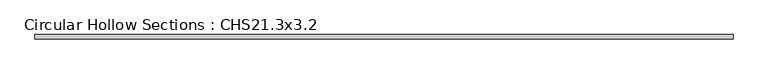
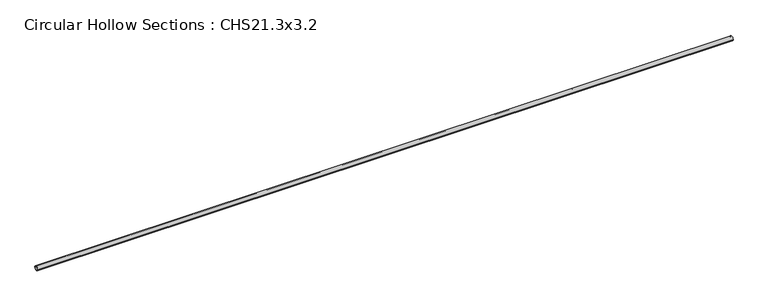
"""IFC4 building model written with IfcOpenShell, lengths in millimetres: member geometry, Circular Hollow Sections : CHS21.3x3.2."""

from ifc_helpers import new_model, si_unit, point, frame, origin, origin_2d, place, context, project, spatial, circle_curve, trimmed, segment, composite_curve, outline, extrude, source, transform, mapped, element, save


def circular_hollow_sections_chs21_3x3_2_132da75c(model_context):
    return source(origin(), model_context, "Body", "SweptSolid", [
        extrude(outline(composite_curve([segment(trimmed(circle_curve(origin_2d(), 10.65), [point((-10.65, 0.0))], [point((10.65, 0.0))], False, "CARTESIAN"), True, "CONTINUOUS"), segment(trimmed(circle_curve(origin_2d(), 10.65), [point((10.65, 0.0))], [point((-10.65, 0.0))], False, "CARTESIAN"), True, "CONTINUOUS")], self_intersect=False), holes=[composite_curve([segment(trimmed(circle_curve(origin_2d(), 7.45), [point((7.45, 0.0))], [point((-7.45, 0.0))], True, "CARTESIAN"), True, "CONTINUOUS"), segment(trimmed(circle_curve(origin_2d(), 7.45), [point((-7.45, 0.0))], [point((7.45, 0.0))], True, "CARTESIAN"), True, "CONTINUOUS")], self_intersect=False)]), frame((-1569.15, 0.0, 0.0), z_axis=(1.0, 0.0, 0.0), x_axis=(0.0, 1.0, 0.0)), (0.0, 0.0, 1.0), 3258.2),
    ])


if __name__ == "__main__":
    model = new_model("IFC4")
    model_context = context("Model", 3, world=origin())
    ifc_project = project(units=[si_unit("LENGTHUNIT", "METRE", prefix="MILLI")], contexts=[model_context])
    site = spatial("IfcSite", under=ifc_project)
    building = spatial("IfcBuilding", under=site)
    placement = place(None, origin())
    circular_hollow_sections_chs21_3x3_2_shape = circular_hollow_sections_chs21_3x3_2_132da75c(model_context)
    element("IfcMember", 1, ObjectType="Circular Hollow Sections : CHS21.3x3.2", at=placement, inside=building, context=model_context, shape_type="MappedRepresentation", body=[
        mapped(circular_hollow_sections_chs21_3x3_2_shape, transform((0.0, 0.0, 0.0), x_axis=(1.0, 0.0, 0.0), y_axis=(0.0, 1.0, 0.0), z_axis=(0.0, 0.0, 1.0))),
    ])
    save(model, "model.ifc")

# Revit data of these elements
# Type "Circular Hollow Sections : CHS21.3x3.2"
#   Section Name Key = "Ch21.3x3.2"
#   Wall Nominal Thickness = 0.32 cm
#   Wall Design Thickness = 0.32 cm
#   Torsional Moment of Inertia = 1.54 cm⁴
#   Torsional Modulus = 1.44 cm³
#   Section Area = 1.82 cm²
#   Plastic Modulus strong axis = 1.06 cm³
#   Perimeter = 0.067 m²/m
#   Nominal Weight = 1.42999 kgf/m
#   Moment of Inertia strong axis = 0.768 cm⁴
#   Length [instance default] = 1500 mm
#   Elastic Modulus strong axis = 0.722 cm³
#   Diameter = 2.13 cm
#   Centroid Vertical = 1.065 cm
#   Centroid Horizontal = 1.065 cm
#   Structural Material [instance default] = Metal - Steel 50-355
#   Type Comments = ""
#   Assembly Code = ""
# Element 1 (IfcMember, "Circular Hollow Sections : CHS21.3x3.2")
#   Structural Material = Metal - Steel 43-275
#   Materials on its faces: "Metal - Steel 43-275"
# Materials
#   "Metal - Steel 50-355": class "Metal", colour RGB 247 247 247, transparency 0, Cost = 0
#   "Metal - Steel 43-275": class "Metal", colour RGB 247 247 247, transparency 0, Cost = 0
